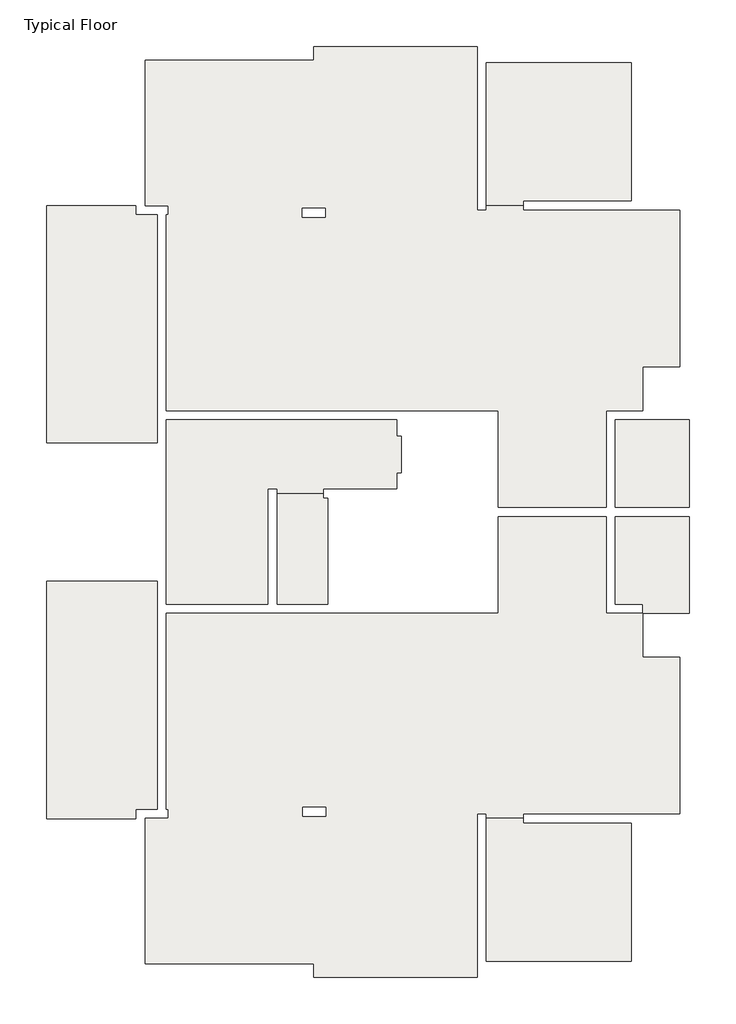
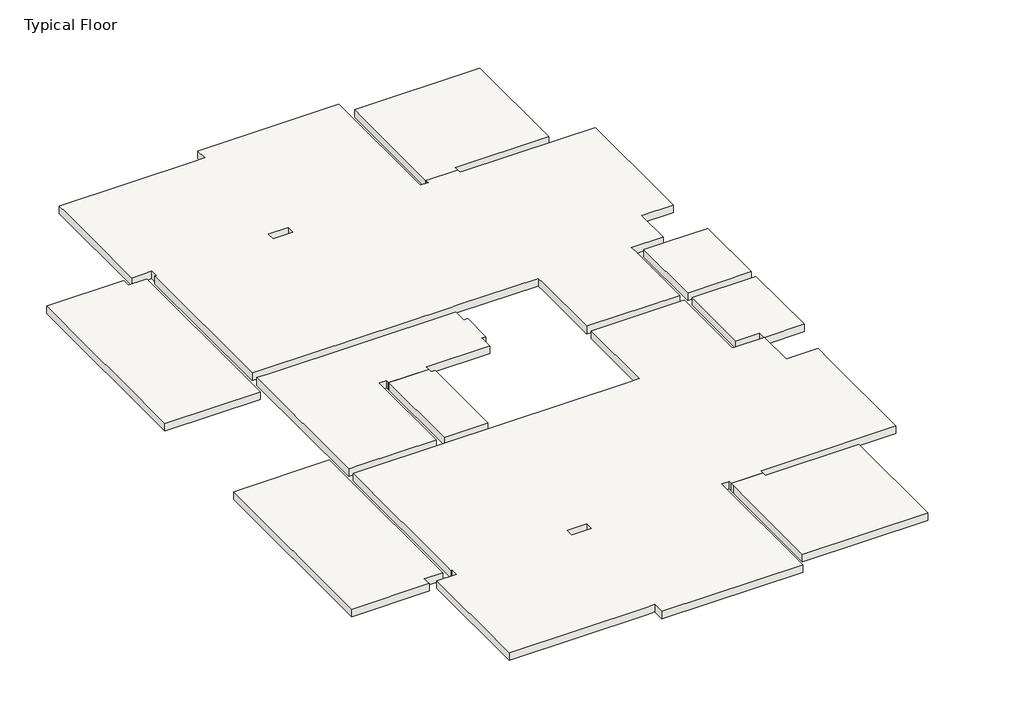
# One storey: 10 slabs.
"""IFC4 building model written with IfcOpenShell, lengths in millimetres."""

import ifcopenshell
import ifcopenshell.guid

model = None  # the IFC model being written
_history = None  # IfcOwnerHistory: only IFC2X3 demands one
_inside = {}  # id of a spatial element -> (the spatial element, [elements in it])
_under = {}  # id of a project, library or spatial element -> (it, [spatial elements below it])
_declared = {}  # id of a project -> (the project, [libraries it declares])
_typed = {}  # id of a type object -> (the type object, [elements of that type])
_made_of = {}  # id of a material, layer set ... -> (it, [elements and type objects made of it])


def new_model(schema):
    """Start an empty IFC model of exactly this schema.

    Asked for "IFC4X3", IfcOpenShell would pick the latest addendum, in which some entities
    have other attributes; the version numbers below select the first issue.
    IFC2X3 requires an IfcOwnerHistory on every rooted entity: one is made here for all.
    """
    global model, _history
    if schema == "IFC4X3":
        model = ifcopenshell.file(schema_version=(4, 3, 0, 0))
    else:
        model = ifcopenshell.file(schema=schema)
    _inside.clear()
    _under.clear()
    _declared.clear()
    _typed.clear()
    _made_of.clear()
    _history = None
    if model.schema == "IFC2X3":
        org = make("IfcOrganization", Name="unknown")
        user = make(
            "IfcPersonAndOrganization",
            ThePerson=make("IfcPerson", FamilyName="unknown"),
            TheOrganization=org,
        )
        app = make(
            "IfcApplication",
            ApplicationDeveloper=org,
            Version="unknown",
            ApplicationFullName="unknown",
            ApplicationIdentifier="unknown",
        )
        _history = make(
            "IfcOwnerHistory",
            OwningUser=user,
            OwningApplication=app,
            ChangeAction="ADDED",
            CreationDate=0,
        )
    return model


def make(cls, **values):
    """One entity of the class cls with the attributes given. An attribute that is None is left unset."""
    return model.create_entity(
        cls, **{name: value for name, value in values.items() if value is not None}
    )


def rooted(cls, **values):
    """An entity with a GlobalId (a new one), such as an element, a storey or a relation."""
    return make(cls, GlobalId=ifcopenshell.guid.new(), OwnerHistory=_history, **values)


def si_unit(unit_type, name, prefix=None):
    """IfcSIUnit, for example si_unit("LENGTHUNIT", "METRE", prefix="MILLI")."""
    return make("IfcSIUnit", UnitType=unit_type, Prefix=prefix, Name=name)


def assignment(units):
    """IfcUnitAssignment: the units of a project."""
    return None if units is None else make("IfcUnitAssignment", Units=units)


def point(xyz):
    """IfcCartesianPoint."""
    return None if xyz is None else make("IfcCartesianPoint", Coordinates=xyz)


def direction(xyz):
    """IfcDirection."""
    return None if xyz is None else make("IfcDirection", DirectionRatios=xyz)


def frame(location, z_axis=None, x_axis=None):
    """IfcAxis2Placement3D, a coordinate frame: its origin and axes. An axis left out is left unset."""
    return make(
        "IfcAxis2Placement3D",
        Location=point(location),
        Axis=direction(z_axis),
        RefDirection=direction(x_axis),
    )


def origin():
    """The frame at (0, 0, 0) with its axes left unset."""
    return frame((0.0, 0.0, 0.0))


def place(relative_to, where):
    """IfcLocalPlacement: puts the frame where relative to a parent placement (None: the world)."""
    return make(
        "IfcLocalPlacement", PlacementRelTo=relative_to, RelativePlacement=where
    )


def context(
    kind, dimensions, precision=None, world=None, true_north=None, identifier=None
):
    """IfcGeometricRepresentationContext, for example the 3D "Model" context."""
    return make(
        "IfcGeometricRepresentationContext",
        ContextIdentifier=identifier,
        ContextType=kind,
        CoordinateSpaceDimension=dimensions,
        Precision=precision,
        WorldCoordinateSystem=world,
        TrueNorth=true_north,
    )


def project(units=None, contexts=None):
    """IfcProject with its units and contexts."""
    return rooted(
        "IfcProject",
        Name="project",
        RepresentationContexts=contexts,
        UnitsInContext=assignment(units),
    )


def spatial(cls, under=None, at=None, **own):
    """A site, building, storey or space (cls), placed at a placement, below another one or the project."""
    s = rooted(cls, ObjectPlacement=at, **own)
    if under is not None:
        _under.setdefault(under.id(), (under, []))[1].append(s)
    return s


def polyline(points):
    """IfcPolyline through the points."""
    return make("IfcPolyline", Points=[point(p) for p in points])


def outline(outer, holes=None, kind="AREA"):
    """IfcArbitraryClosedProfileDef: a profile drawn as a closed curve; with holes, ...WithVoids."""
    if holes is None:
        return make("IfcArbitraryClosedProfileDef", ProfileType=kind, OuterCurve=outer)
    return make(
        "IfcArbitraryProfileDefWithVoids",
        ProfileType=kind,
        OuterCurve=outer,
        InnerCurves=holes,
    )


def extrude(swept, where, along, depth):
    """IfcExtrudedAreaSolid: the profile swept, set in the frame where, extruded along a direction by depth."""
    return make(
        "IfcExtrudedAreaSolid",
        SweptArea=swept,
        Position=where,
        ExtrudedDirection=direction(along),
        Depth=depth,
    )


def faces_of(points, faces, orient=None, outer=None):
    """IfcFace entities. A face is a list of loops; a loop is a list of indices into points, from 0.

    orient and outer hold one flag for each loop. By default every Orientation is true, the
    first loop of a face is its IfcFaceOuterBound and the others are IfcFaceBound.
    """
    made = []
    for i, loops in enumerate(faces):
        bounds = []
        for j, loop in enumerate(loops):
            is_outer = j == 0 if outer is None else outer[i][j]
            bounds.append(
                make(
                    "IfcFaceOuterBound" if is_outer else "IfcFaceBound",
                    Bound=make("IfcPolyLoop", Polygon=[points[k] for k in loop]),
                    Orientation=True if orient is None else orient[i][j],
                )
            )
        made.append(make("IfcFace", Bounds=bounds))
    return made


def faceted_brep(points, faces, orient=None, outer=None, voids=None):
    """IfcFacetedBrep: a solid bounded by flat faces; with voids (closed shells), ...WithVoids."""
    shared = [point(p) for p in points]
    hull = make("IfcClosedShell", CfsFaces=faces_of(shared, faces, orient, outer))
    if voids is None:
        return make("IfcFacetedBrep", Outer=hull)
    return make(
        "IfcFacetedBrepWithVoids",
        Outer=hull,
        Voids=[
            make(cls, CfsFaces=faces_of(shared, fs, o, b)) for cls, fs, o, b in voids
        ],
    )


def shape(context_of_items, identifier, shape_type, items):
    """IfcShapeRepresentation: the items that make up one representation, for example the "Body"."""
    return make(
        "IfcShapeRepresentation",
        ContextOfItems=context_of_items,
        RepresentationIdentifier=identifier,
        RepresentationType=shape_type,
        Items=items,
    )


def made_of(thing, what):
    """Note that an element or type object is made of a material, layer set ...; save() writes the relation."""
    if what is not None:
        _made_of.setdefault(what.id(), (what, []))[1].append(thing)
    return thing


def element(
    cls,
    number,
    at=None,
    inside=None,
    cuts=None,
    type_object=None,
    material=None,
    context=None,
    identifier="Body",
    shape_type=None,
    held_by="IfcProductDefinitionShape",
    body=None,
    shapes=None,
    **own,
):
    """One element of the class cls, such as IfcWall. Its Tag is "e" and its number.

    at: its placement. inside: the storey or other place that contains it. cuts: it is an
    opening in that element (IfcRelVoidsElement). A single representation is given by context,
    identifier, shape_type and body (its items); several are given by shapes. held_by: the class
    of the entity that holds the representations. save() writes the other relations.
    """
    e = rooted(cls, Tag="e%d" % number, ObjectPlacement=at, **own)
    if body is not None:
        shapes = [shape(context, identifier, shape_type, body)]
    if shapes is not None:
        e.Representation = make(held_by, Representations=shapes)
    if inside is not None:
        _inside.setdefault(inside.id(), (inside, []))[1].append(e)
    if cuts is not None:
        rooted(
            "IfcRelVoidsElement", RelatingBuildingElement=cuts, RelatedOpeningElement=e
        )
    if type_object is not None:
        _typed.setdefault(type_object.id(), (type_object, []))[1].append(e)
    return made_of(e, material)


def aggregate(whole, parts):
    """IfcRelAggregates: a whole, such as a stair, and the parts it consists of."""
    return rooted("IfcRelAggregates", RelatingObject=whole, RelatedObjects=parts)


def save(model, path):
    """Write the relations noted so far, then the file.

    IfcRelAggregates (storeys below a building ...), IfcRelContainedInSpatialStructure (elements
    in a storey), IfcRelDefinesByType, IfcRelAssociatesMaterial and IfcRelDeclares: one each for
    every whole, place, type object, material and project.
    """
    for whole, parts in _under.values():
        aggregate(whole, parts)
    for where, things in _inside.values():
        rooted(
            "IfcRelContainedInSpatialStructure",
            RelatedElements=things,
            RelatingStructure=where,
        )
    for kind, things in _typed.values():
        rooted("IfcRelDefinesByType", RelatedObjects=things, RelatingType=kind)
    for what, things in _made_of.values():
        rooted("IfcRelAssociatesMaterial", RelatedObjects=things, RelatingMaterial=what)
    for by, libraries in _declared.values():
        rooted("IfcRelDeclares", RelatingContext=by, RelatedDefinitions=libraries)
    model.write(path)


model = new_model("IFC4")

# Units and contexts
model_context = context("Model", 3, world=origin())
ifc_project = project(units=[si_unit("LENGTHUNIT", "METRE", prefix="MILLI")], contexts=[model_context])

# Site, building, storey
site = spatial("IfcSite", under=ifc_project)
building = spatial("IfcBuilding", under=site)
storey = spatial("IfcBuildingStorey", under=building, Name="Typical Floor", Elevation=3000.0)

# Slabs
placement = place(None, origin())
element("IfcSlab", 1, ObjectType="20", at=placement, inside=storey, context=model_context, shape_type="Brep", body=[
    faceted_brep([(-1086.1844466, 16787.4100295, 2800.0), (-1086.1844466, 11837.4100295, 2800.0), (-3487.6312201, 11837.4100295, 2800.0), (-3487.6312201, 16987.4100295, 2800.0), (-1547.6312201, 16987.4100295, 2800.0), (-1547.6312201, 16787.4100295, 2800.0), (-1086.1844466, 11837.4100295, 3000.0), (-1086.1844466, 12337.0195651, 3000.0), (-1086.1844466, 12537.0195651, 3000.0), (-1086.1844466, 16787.4100295, 3000.0), (-1547.6312201, 16787.4100295, 3000.0), (-1547.6312201, 16987.4100295, 3000.0), (-3487.6312201, 16987.4100295, 3000.0), (-3487.6312201, 11837.4100295, 3000.0)], [[[0, 1, 2, 3, 4, 5]], [[6, 7, 8, 9, 10, 11, 12, 13]], [[1, 0, 9, 8, 7, 6]], [[2, 1, 6, 13]], [[3, 2, 13, 12]], [[4, 3, 12, 11]], [[5, 4, 11, 10]], [[0, 5, 10, 9]]]),
])
element("IfcSlab", 2, ObjectType="20", at=placement, inside=storey, context=model_context, shape_type="Brep", body=[
    faceted_brep([(-1086.1844466, 8836.9784636, 2800.0), (-1086.1844466, 3886.9784636, 2800.0), (-1547.6312201, 3886.9784636, 2800.0), (-1547.6312201, 3686.9784636, 2800.0), (-1547.6312201, 3686.5951919, 2800.0), (-3487.6312201, 3686.5951919, 2800.0), (-3487.6312201, 8836.9784636, 2800.0), (-1086.1844466, 3886.9784636, 3000.0), (-1086.1844466, 8136.34139, 3000.0), (-1086.1844466, 8336.34139, 3000.0), (-1086.1844466, 8836.9784636, 3000.0), (-3487.6312201, 8836.9784636, 3000.0), (-3487.6312201, 3686.5951919, 3000.0), (-1547.6312201, 3686.5951919, 3000.0), (-1547.6312201, 3686.9784636, 3000.0), (-1547.6312201, 3886.9784636, 3000.0)], [[[0, 1, 2, 3, 4, 5, 6]], [[7, 8, 9, 10, 11, 12, 13, 14, 15]], [[1, 0, 10, 9, 8, 7]], [[0, 6, 11, 10]], [[6, 5, 12, 11]], [[5, 4, 13, 12]], [[2, 15, 14, 13, 4, 3]], [[2, 1, 7, 15]]]),
])
element("IfcSlab", 3, ObjectType="20", at=placement, inside=storey, context=model_context, shape_type="Brep", body=[
    faceted_brep([(9452.8825489, 7186.4846031, 2800.0), (10255.2882967, 7186.4846031, 2800.0), (10255.2882967, 7158.0471031, 2800.0), (10255.2882967, 3786.4646946, 2800.0), (9453.0058534, 3786.4646946, 2800.0), (6853.6634778, 3786.4646946, 2800.0), (6853.6634778, 3691.2119202, 2800.0), (6055.3348071, 3691.2119202, 2800.0), (6055.3348071, 3786.4646946, 2800.0), (5855.2115026, 3786.4646946, 2800.0), (5855.2115026, 336.1975347, 2800.0), (5855.2115026, 237.7388417, 2800.0), (2314.1854671, 237.7388417, 2800.0), (2314.1854671, 537.7388417, 2800.0), (2114.3087716, 537.7388417, 2800.0), (-1347.7545247, 537.7388417, 2800.0), (-1347.7545247, 3686.9784636, 2800.0), (-847.7545247, 3686.9784636, 2800.0), (-847.7545247, 3886.9784636, 2800.0), (-886.3077512, 3886.9784636, 2800.0), (-886.3077512, 8136.34139, 2800.0), (-586.1844466, 8136.34139, 2800.0), (1314.1854671, 8136.34139, 2800.0), (6113.8977564, 8136.34139, 2800.0), (6313.7744519, 8136.34139, 2800.0), (6313.7744519, 10238.2526107, 2800.0), (8652.7592443, 10238.2526107, 2800.0), (8652.7592443, 8336.34139, 2800.0), (8652.7592443, 8136.34139, 2800.0), (9452.8825489, 8136.34139, 2800.0), (2066.6823845, 3734.6356769, 2800.0), (2566.6823845, 3734.6356769, 2800.0), (2566.6823845, 3934.6356769, 2800.0), (2066.6823845, 3934.6356769, 2800.0), (10255.2882967, 7186.4846031, 3000.0), (9452.8825489, 7186.4846031, 3000.0), (9452.8825489, 8136.34139, 3000.0), (8652.7592443, 8136.34139, 3000.0), (8652.7592443, 8336.34139, 3000.0), (8652.7592443, 10238.2526107, 3000.0), (6313.7744519, 10238.2526107, 3000.0), (6313.7744519, 8136.34139, 3000.0), (6113.8977564, 8136.34139, 3000.0), (1314.1854671, 8136.34139, 3000.0), (-586.1844466, 8136.34139, 3000.0), (-886.3077512, 8136.34139, 3000.0), (-886.3077512, 3886.9784636, 3000.0), (-847.7545247, 3886.9784636, 3000.0), (-847.7545247, 3686.9784636, 3000.0), (-1347.7545247, 3686.9784636, 3000.0), (-1347.7545247, 836.1975347, 3000.0), (-1347.7545247, 537.7388417, 3000.0), (2114.3087716, 537.7388417, 3000.0), (2314.1854671, 537.7388417, 3000.0), (2314.1854671, 237.7388417, 3000.0), (5855.2115026, 237.7388417, 3000.0), (5855.2115026, 336.1975347, 3000.0), (5855.2115026, 3786.4646946, 3000.0), (6055.3348071, 3786.4646946, 3000.0), (6055.3348071, 3691.2119202, 3000.0), (6853.6634778, 3691.2119202, 3000.0), (6853.6634778, 3786.4646946, 3000.0), (9453.0058534, 3786.4646946, 3000.0), (10255.2882967, 3786.4646946, 3000.0), (10255.2882967, 6686.3824915, 3000.0), (10255.2882967, 7158.0471031, 3000.0), (2566.6823845, 3734.6356769, 3000.0), (2066.6823845, 3734.6356769, 3000.0), (2066.6823845, 3934.6356769, 3000.0), (2566.6823845, 3934.6356769, 3000.0)], [[[0, 1, 2, 3, 4, 5, 6, 7, 8, 9, 10, 11, 12, 13, 14, 15, 16, 17, 18, 19, 20, 21, 22, 23, 24, 25, 26, 27, 28, 29], [30, 31, 32, 33]], [[34, 35, 36, 37, 38, 39, 40, 41, 42, 43, 44, 45, 46, 47, 48, 49, 50, 51, 52, 53, 54, 55, 56, 57, 58, 59, 60, 61, 62, 63, 64, 65], [66, 67, 68, 69]], [[1, 0, 35, 34]], [[2, 1, 34, 65]], [[3, 2, 65, 64, 63]], [[3, 63, 62, 61, 5, 4]], [[6, 5, 61, 60]], [[7, 6, 60, 59]], [[8, 7, 59, 58]], [[9, 8, 58, 57]], [[9, 57, 56, 55, 11, 10]], [[12, 11, 55, 54]], [[13, 12, 54, 53]], [[13, 53, 52, 51, 15, 14]], [[16, 15, 51, 50, 49]], [[17, 16, 49, 48]], [[18, 17, 48, 47]], [[19, 18, 47, 46]], [[20, 19, 46, 45]], [[20, 45, 44, 43, 42, 41, 24, 23, 22, 21]], [[25, 24, 41, 40]], [[26, 25, 40, 39]], [[26, 39, 38, 37, 28, 27]], [[29, 28, 37, 36]], [[0, 29, 36, 35]], [[30, 67, 66, 31]], [[67, 30, 33, 68]], [[68, 33, 32, 69]], [[69, 32, 31, 66]]]),
])
element("IfcSlab", 4, ObjectType="20", at=placement, inside=storey, context=model_context, shape_type="SweptSolid", body=[
    extrude(outline(polyline([(9203.0058534, 586.1975347), (6055.3348071, 586.1975347), (6055.3348071, 3586.4646946), (6055.3348071, 3691.2119202), (6853.6634778, 3691.2119202), (6853.6634778, 3586.4646946), (9203.0058534, 3586.4646946), (9203.0058534, 586.1975347)])), frame((0.0, 0.0, 2800.0), z_axis=(0.0, 0.0, 1.0), x_axis=(1.0, 0.0, 0.0)), (0.0, 0.0, 1.0), 200.0),
])
element("IfcSlab", 5, ObjectType="20", at=placement, inside=storey, context=model_context, shape_type="Brep", body=[
    faceted_brep([(9452.8825489, 12537.0195651, 2800.0), (8652.8825489, 12537.0195651, 2800.0), (8652.8825489, 12337.0195651, 2800.0), (8652.8825489, 10438.2526107, 2800.0), (6313.8977564, 10438.2526107, 2800.0), (6313.8977564, 12337.0195651, 2800.0), (6313.8977564, 12537.0195651, 2800.0), (4314.617033, 12537.0195651, 2800.0), (4114.617033, 12537.0195651, 2800.0), (-586.1844466, 12537.0195651, 2800.0), (-886.1844466, 12537.0195651, 2800.0), (-886.1844466, 16787.4100295, 2800.0), (-847.6312201, 16787.4100295, 2800.0), (-847.6312201, 16987.4100295, 2800.0), (-1347.6312201, 16987.4100295, 2800.0), (-1347.6312201, 20138.1909584, 2800.0), (2113.2812336, 20138.1909584, 2800.0), (2313.2812336, 20138.1909584, 2800.0), (2313.2812336, 20438.1909584, 2800.0), (5855.3348071, 20438.1909584, 2800.0), (5855.3348071, 20337.1634204, 2800.0), (5855.3348071, 16886.8962605, 2800.0), (6055.3348071, 16886.8962605, 2800.0), (6055.3348071, 16986.8962605, 2800.0), (6853.6634778, 16986.8962605, 2800.0), (6853.6634778, 16886.8962605, 2800.0), (9453.0058534, 16886.8962605, 2800.0), (10255.2560168, 16886.8962605, 2800.0), (10255.2560168, 13485.039794, 2800.0), (9452.8825489, 13485.039794, 2800.0), (2563.507292, 16933.4642836, 2800.0), (2063.507292, 16933.4642836, 2800.0), (2063.507292, 16733.4642836, 2800.0), (2563.507292, 16733.4642836, 2800.0), (8652.8825489, 12537.0195651, 3000.0), (9452.8825489, 12537.0195651, 3000.0), (9452.8825489, 13485.039794, 3000.0), (10255.2560168, 13485.039794, 3000.0), (10255.2560168, 13985.039794, 3000.0), (10255.2560168, 16886.8962605, 3000.0), (9453.0058534, 16886.8962605, 3000.0), (6853.6634778, 16886.8962605, 3000.0), (6853.6634778, 16986.8962605, 3000.0), (6055.3348071, 16986.8962605, 3000.0), (6055.3348071, 16886.8962605, 3000.0), (5855.3348071, 16886.8962605, 3000.0), (5855.3348071, 20337.1634204, 3000.0), (5855.3348071, 20438.1909584, 3000.0), (2313.2812336, 20438.1909584, 3000.0), (2313.2812336, 20138.1909584, 3000.0), (2113.2812336, 20138.1909584, 3000.0), (-1347.6312201, 20138.1909584, 3000.0), (-1347.6312201, 19838.1909584, 3000.0), (-1347.6312201, 16987.4100295, 3000.0), (-847.6312201, 16987.4100295, 3000.0), (-847.6312201, 16787.4100295, 3000.0), (-886.1844466, 16787.4100295, 3000.0), (-886.1844466, 12537.0195651, 3000.0), (-586.1844466, 12537.0195651, 3000.0), (4114.617033, 12537.0195651, 3000.0), (4314.617033, 12537.0195651, 3000.0), (6313.8977564, 12537.0195651, 3000.0), (6313.8977564, 12337.0195651, 3000.0), (6313.8977564, 10438.2526107, 3000.0), (8652.8825489, 10438.2526107, 3000.0), (8652.8825489, 12337.0195651, 3000.0), (2063.507292, 16933.4642836, 3000.0), (2563.507292, 16933.4642836, 3000.0), (2563.507292, 16733.4642836, 3000.0), (2063.507292, 16733.4642836, 3000.0)], [[[0, 1, 2, 3, 4, 5, 6, 7, 8, 9, 10, 11, 12, 13, 14, 15, 16, 17, 18, 19, 20, 21, 22, 23, 24, 25, 26, 27, 28, 29], [30, 31, 32, 33]], [[34, 35, 36, 37, 38, 39, 40, 41, 42, 43, 44, 45, 46, 47, 48, 49, 50, 51, 52, 53, 54, 55, 56, 57, 58, 59, 60, 61, 62, 63, 64, 65], [66, 67, 68, 69]], [[1, 0, 35, 34]], [[29, 28, 37, 36]], [[0, 29, 36, 35]], [[1, 34, 65, 64, 3, 2]], [[4, 3, 64, 63]], [[4, 63, 62, 61, 6, 5]], [[6, 61, 60, 59, 58, 57, 10, 9, 8, 7]], [[11, 10, 57, 56]], [[12, 11, 56, 55]], [[13, 12, 55, 54]], [[14, 13, 54, 53]], [[15, 14, 53, 52, 51]], [[15, 51, 50, 49, 17, 16]], [[18, 17, 49, 48]], [[19, 18, 48, 47]], [[19, 47, 46, 45, 21, 20]], [[22, 21, 45, 44]], [[23, 22, 44, 43]], [[24, 23, 43, 42]], [[25, 24, 42, 41]], [[26, 25, 41, 40]], [[27, 26, 40, 39]], [[28, 27, 39, 38, 37]], [[30, 67, 66, 31]], [[67, 30, 33, 68]], [[68, 33, 32, 69]], [[69, 32, 31, 66]]]),
])
element("IfcSlab", 6, ObjectType="20", at=placement, inside=storey, context=model_context, shape_type="SweptSolid", body=[
    extrude(outline(polyline([(6853.6634778, 16986.8962605), (6055.3348071, 16986.8962605), (6055.3348071, 20087.1634204), (9203.0058534, 20087.1634204), (9203.0058534, 17086.8962605), (6853.6634778, 17086.8962605), (6853.6634778, 16986.8962605)])), frame((0.0, 0.0, 2800.0), z_axis=(0.0, 0.0, 1.0), x_axis=(1.0, 0.0, 0.0)), (0.0, 0.0, 1.0), 200.0),
])
element("IfcSlab", 7, ObjectType="20", at=placement, inside=storey, context=model_context, shape_type="Brep", body=[
    faceted_brep([(1314.1854671, 8336.34139, 2800.0), (-886.1844466, 8336.34139, 2800.0), (-886.1844466, 12337.0195651, 2800.0), (4114.617033, 12337.0195651, 2800.0), (4114.617033, 11986.6702022, 2800.0), (4214.617033, 11986.6702022, 2800.0), (4214.617033, 11186.5468976, 2800.0), (4114.617033, 11186.5468976, 2800.0), (4114.617033, 10837.286725, 2800.0), (2514.3704239, 10837.286725, 2800.0), (2514.3704239, 10757.286725, 2800.0), (2514.3704239, 10737.286725, 2800.0), (1514.1854671, 10737.286725, 2800.0), (1514.1854671, 10757.286725, 2800.0), (1514.1854671, 10837.286725, 2800.0), (1314.1854671, 10837.286725, 2800.0), (-886.1844466, 8336.34139, 3000.0), (-586.1844466, 8336.34139, 3000.0), (1314.1854671, 8336.34139, 3000.0), (1314.1854671, 10837.286725, 3000.0), (1514.1854671, 10837.286725, 3000.0), (1514.1854671, 10757.286725, 3000.0), (1514.1854671, 10737.286725, 3000.0), (2514.3704239, 10737.286725, 3000.0), (2514.3704239, 10757.286725, 3000.0), (2514.3704239, 10837.286725, 3000.0), (4114.617033, 10837.286725, 3000.0), (4114.617033, 11186.5468976, 3000.0), (4214.617033, 11186.5468976, 3000.0), (4214.617033, 11986.6702022, 3000.0), (4114.617033, 11986.6702022, 3000.0), (4114.617033, 12337.0195651, 3000.0), (-586.1844466, 12337.0195651, 3000.0), (-886.1844466, 12337.0195651, 3000.0)], [[[0, 1, 2, 3, 4, 5, 6, 7, 8, 9, 10, 11, 12, 13, 14, 15]], [[16, 17, 18, 19, 20, 21, 22, 23, 24, 25, 26, 27, 28, 29, 30, 31, 32, 33]], [[1, 0, 18, 17, 16]], [[2, 1, 16, 33]], [[3, 2, 33, 32, 31]], [[4, 3, 31, 30]], [[5, 4, 30, 29]], [[6, 5, 29, 28]], [[7, 6, 28, 27]], [[8, 7, 27, 26]], [[9, 8, 26, 25]], [[10, 9, 25, 24]], [[11, 10, 24, 23]], [[12, 11, 23, 22]], [[13, 12, 22, 21]], [[14, 13, 21, 20]], [[15, 14, 20, 19]], [[0, 15, 19, 18]]]),
])
element("IfcSlab", 8, ObjectType="20", at=placement, inside=storey, context=model_context, shape_type="Brep", body=[
    faceted_brep([(8852.561957, 8336.34139, 2800.0), (8852.561957, 10238.2526107, 2800.0), (8852.8825489, 10238.2526107, 2800.0), (10453.8977564, 10238.2526107, 2800.0), (10453.8977564, 8136.34139, 2800.0), (9452.8825489, 8136.34139, 2800.0), (9452.8825489, 8336.34139, 2800.0), (8852.8825489, 8336.34139, 2800.0), (8852.561957, 10238.2526107, 3000.0), (8852.561957, 8336.34139, 3000.0), (9452.8825489, 8336.34139, 3000.0), (9452.8825489, 8136.34139, 3000.0), (10453.8977564, 8136.34139, 3000.0), (10453.8977564, 10238.2526107, 3000.0), (8852.8825489, 10238.2526107, 3000.0)], [[[0, 1, 2, 3, 4, 5, 6, 7]], [[8, 9, 10, 11, 12, 13, 14]], [[4, 12, 11, 5]], [[9, 0, 7, 6, 10]], [[1, 0, 9, 8]], [[3, 2, 1, 8, 14, 13]], [[4, 3, 13, 12]], [[10, 6, 5, 11]]]),
])
element("IfcSlab", 9, ObjectType="20", at=placement, inside=storey, context=model_context, shape_type="Brep", body=[
    faceted_brep([(10453.8977564, 12337.0195651, 2800.0), (10453.8977564, 10438.2526107, 2800.0), (8852.8825489, 10438.2526107, 2800.0), (8852.8825489, 12337.0195651, 2800.0), (10453.8977564, 10438.2526107, 3000.0), (10453.8977564, 12337.0195651, 3000.0), (9452.8825489, 12337.0195651, 3000.0), (8852.8825489, 12337.0195651, 3000.0), (8852.8825489, 10438.2526107, 3000.0)], [[[0, 1, 2, 3]], [[4, 5, 6, 7, 8]], [[1, 0, 5, 4]], [[2, 1, 4, 8]], [[3, 2, 8, 7]], [[0, 3, 7, 6, 5]]]),
])
element("IfcSlab", 10, ObjectType="20", at=placement, inside=storey, context=model_context, shape_type="SweptSolid", body=[
    extrude(outline(polyline([(2619.3704239, 8336.34139), (1514.1854671, 8336.34139), (1514.1854671, 10737.286725), (2514.3704239, 10737.286725), (2514.3704239, 10637.286725), (2619.3704239, 10637.286725), (2619.3704239, 8336.34139)])), frame((0.0, 0.0, 2800.0), z_axis=(0.0, 0.0, 1.0), x_axis=(1.0, 0.0, 0.0)), (0.0, 0.0, 1.0), 200.0),
])

save(model, "model.ifc")

# Revit data of these elements
# Type "20"
#   Function = 0
#   Layers, outside or top first: 20 cm "Concrete" (function 1)
# Element 1 (IfcSlab, "20")
#   Mark = "S1"
#   SOFiSTiK_AMG_Comments = ""
#   built-in parameter 1001955 = 1.5708 (stored number, unit not read)
#   Height Offset From Level = 0 cm
#   built-in parameter 1001954 = 1
#   SOFiSTiK_AMG_Scheduled = yes
#   SOFiSTiK_AMG_Adjusted = yes
#   Phase Created = New Construction
#   Materials on its faces: "Concrete"
# Element 2 (IfcSlab, "20")
#   Mark = "S2"
#   SOFiSTiK_AMG_Comments = ""
#   built-in parameter 1001955 = -1.5708 (stored number, unit not read)
#   Height Offset From Level = 0 cm
#   built-in parameter 1001954 = 1
#   SOFiSTiK_AMG_Scheduled = yes
#   SOFiSTiK_AMG_Adjusted = yes
#   Phase Created = New Construction
#   Materials on its faces: "Concrete"
# Element 3 (IfcSlab, "20")
#   Mark = "S3"
#   SOFiSTiK_AMG_Comments = ""
#   built-in parameter 1001955 = -1.5708 (stored number, unit not read)
#   Height Offset From Level = 0 cm
#   built-in parameter 1001954 = 1
#   SOFiSTiK_AMG_Scheduled = yes
#   SOFiSTiK_AMG_Adjusted = no
#   Phase Created = New Construction
#   Materials on its faces: "Concrete"
# Element 4 (IfcSlab, "20")
#   Mark = "S4"
#   SOFiSTiK_AMG_Comments = ""
#   Height Offset From Level = 0 cm
#   built-in parameter 1001954 = 1
#   SOFiSTiK_AMG_Scheduled = yes
#   SOFiSTiK_AMG_Adjusted = yes
#   Phase Created = New Construction
#   Materials on its faces: "Concrete"
# Element 5 (IfcSlab, "20")
#   Mark = "S5"
#   SOFiSTiK_AMG_Comments = ""
#   Height Offset From Level = 0 cm
#   built-in parameter 1001954 = 1
#   SOFiSTiK_AMG_Scheduled = yes
#   SOFiSTiK_AMG_Adjusted = no
#   Phase Created = New Construction
#   Materials on its faces: "Concrete"
# Element 6 (IfcSlab, "20")
#   Mark = "S6"
#   SOFiSTiK_AMG_Comments = ""
#   Height Offset From Level = 0 cm
#   built-in parameter 1001954 = 1
#   SOFiSTiK_AMG_Scheduled = yes
#   SOFiSTiK_AMG_Adjusted = yes
#   Phase Created = New Construction
#   Materials on its faces: "Concrete"
# Element 7 (IfcSlab, "20")
#   Mark = "S7"
#   SOFiSTiK_AMG_Comments = ""
#   Height Offset From Level = 0 cm
#   built-in parameter 1001954 = 1
#   SOFiSTiK_AMG_Scheduled = yes
#   SOFiSTiK_AMG_Adjusted = no
#   Phase Created = New Construction
#   Materials on its faces: "Concrete"
# Element 8 (IfcSlab, "20")
#   Mark = "S8"
#   SOFiSTiK_AMG_Comments = ""
#   Height Offset From Level = 0 cm
#   built-in parameter 1001954 = 1
#   SOFiSTiK_AMG_Scheduled = yes
#   SOFiSTiK_AMG_Adjusted = yes
#   Phase Created = New Construction
#   Materials on its faces: "Concrete"
# Element 9 (IfcSlab, "20")
#   Mark = "S9"
#   SOFiSTiK_AMG_Comments = ""
#   Height Offset From Level = 0 cm
#   built-in parameter 1001954 = 1
#   SOFiSTiK_AMG_Scheduled = yes
#   SOFiSTiK_AMG_Adjusted = yes
#   Phase Created = New Construction
#   Materials on its faces: "Concrete"
# Element 10 (IfcSlab, "20")
#   Mark = "S10"
#   SOFiSTiK_AMG_Comments = ""
#   Height Offset From Level = 0 cm
#   built-in parameter 1001954 = 1
#   SOFiSTiK_AMG_Scheduled = yes
#   SOFiSTiK_AMG_Adjusted = yes
#   Phase Created = New Construction
#   Materials on its faces: "Concrete"
# Materials
#   "Concrete": class "Concrete", colour RGB 192 192 192, transparency 0, Keynote = "01000", Description = "Cast-in-place concrete", Cost = 0
